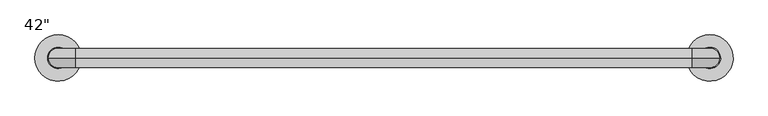
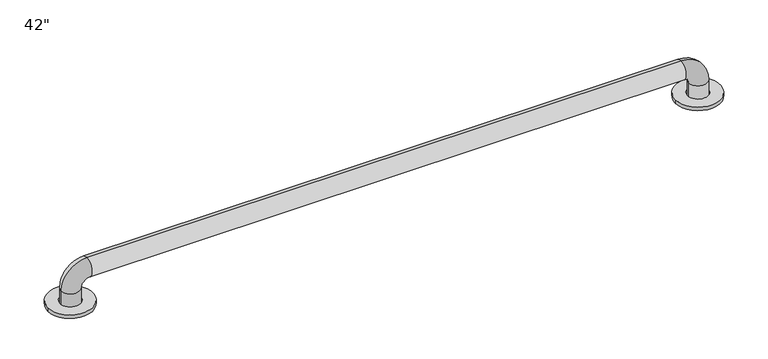
"""IFC4 building model written with IfcOpenShell, lengths in millimetres: proxy geometry."""

import ifcopenshell
import ifcopenshell.guid

model = None  # the IFC model being written
_history = None  # IfcOwnerHistory: only IFC2X3 demands one
_inside = {}  # id of a spatial element -> (the spatial element, [elements in it])
_under = {}  # id of a project, library or spatial element -> (it, [spatial elements below it])
_declared = {}  # id of a project -> (the project, [libraries it declares])
_typed = {}  # id of a type object -> (the type object, [elements of that type])
_made_of = {}  # id of a material, layer set ... -> (it, [elements and type objects made of it])


def new_model(schema):
    """Start an empty IFC model of exactly this schema.

    Asked for "IFC4X3", IfcOpenShell would pick the latest addendum, in which some entities
    have other attributes; the version numbers below select the first issue.
    IFC2X3 requires an IfcOwnerHistory on every rooted entity: one is made here for all.
    """
    global model, _history
    if schema == "IFC4X3":
        model = ifcopenshell.file(schema_version=(4, 3, 0, 0))
    else:
        model = ifcopenshell.file(schema=schema)
    _inside.clear()
    _under.clear()
    _declared.clear()
    _typed.clear()
    _made_of.clear()
    _history = None
    if model.schema == "IFC2X3":
        org = make("IfcOrganization", Name="unknown")
        user = make(
            "IfcPersonAndOrganization",
            ThePerson=make("IfcPerson", FamilyName="unknown"),
            TheOrganization=org,
        )
        app = make(
            "IfcApplication",
            ApplicationDeveloper=org,
            Version="unknown",
            ApplicationFullName="unknown",
            ApplicationIdentifier="unknown",
        )
        _history = make(
            "IfcOwnerHistory",
            OwningUser=user,
            OwningApplication=app,
            ChangeAction="ADDED",
            CreationDate=0,
        )
    return model


def make(cls, **values):
    """One entity of the class cls with the attributes given. An attribute that is None is left unset."""
    return model.create_entity(
        cls, **{name: value for name, value in values.items() if value is not None}
    )


def rooted(cls, **values):
    """An entity with a GlobalId (a new one), such as an element, a storey or a relation."""
    return make(cls, GlobalId=ifcopenshell.guid.new(), OwnerHistory=_history, **values)


def si_unit(unit_type, name, prefix=None):
    """IfcSIUnit, for example si_unit("LENGTHUNIT", "METRE", prefix="MILLI")."""
    return make("IfcSIUnit", UnitType=unit_type, Prefix=prefix, Name=name)


def assignment(units):
    """IfcUnitAssignment: the units of a project."""
    return None if units is None else make("IfcUnitAssignment", Units=units)


def point(xyz):
    """IfcCartesianPoint."""
    return None if xyz is None else make("IfcCartesianPoint", Coordinates=xyz)


def direction(xyz):
    """IfcDirection."""
    return None if xyz is None else make("IfcDirection", DirectionRatios=xyz)


def frame(location, z_axis=None, x_axis=None):
    """IfcAxis2Placement3D, a coordinate frame: its origin and axes. An axis left out is left unset."""
    return make(
        "IfcAxis2Placement3D",
        Location=point(location),
        Axis=direction(z_axis),
        RefDirection=direction(x_axis),
    )


def frame_2d(location, x_axis=None):
    """IfcAxis2Placement2D, a coordinate frame in the plane: its origin and x axis."""
    return make(
        "IfcAxis2Placement2D", Location=point(location), RefDirection=direction(x_axis)
    )


def origin():
    """The frame at (0, 0, 0) with its axes left unset."""
    return frame((0.0, 0.0, 0.0))


def origin_with_axes():
    """The frame at (0, 0, 0) with the z axis (0, 0, 1) and the x axis (1, 0, 0) written out."""
    return frame((0.0, 0.0, 0.0), z_axis=(0.0, 0.0, 1.0), x_axis=(1.0, 0.0, 0.0))


def origin_2d():
    """The frame at (0, 0) in the plane with its x axis left unset."""
    return frame_2d((0.0, 0.0))


def place(relative_to, where):
    """IfcLocalPlacement: puts the frame where relative to a parent placement (None: the world)."""
    return make(
        "IfcLocalPlacement", PlacementRelTo=relative_to, RelativePlacement=where
    )


def context(
    kind, dimensions, precision=None, world=None, true_north=None, identifier=None
):
    """IfcGeometricRepresentationContext, for example the 3D "Model" context."""
    return make(
        "IfcGeometricRepresentationContext",
        ContextIdentifier=identifier,
        ContextType=kind,
        CoordinateSpaceDimension=dimensions,
        Precision=precision,
        WorldCoordinateSystem=world,
        TrueNorth=true_north,
    )


def project(units=None, contexts=None):
    """IfcProject with its units and contexts."""
    return rooted(
        "IfcProject",
        Name="project",
        RepresentationContexts=contexts,
        UnitsInContext=assignment(units),
    )


def spatial(cls, under=None, at=None, **own):
    """A site, building, storey or space (cls), placed at a placement, below another one or the project."""
    s = rooted(cls, ObjectPlacement=at, **own)
    if under is not None:
        _under.setdefault(under.id(), (under, []))[1].append(s)
    return s


def circle_curve(where, radius):
    """IfcCircle in the frame where."""
    return make("IfcCircle", Position=where, Radius=radius)


def ellipse_curve(where, semi_axis1, semi_axis2):
    """IfcEllipse in the frame where."""
    return make(
        "IfcEllipse", Position=where, SemiAxis1=semi_axis1, SemiAxis2=semi_axis2
    )


def trimmed(basis, trim1, trim2, sense, master):
    """IfcTrimmedCurve: the piece of a basis curve between two trims."""
    return make(
        "IfcTrimmedCurve",
        BasisCurve=basis,
        Trim1=trim1,
        Trim2=trim2,
        SenseAgreement=sense,
        MasterRepresentation=master,
    )


def segment(curve, same_sense, transition):
    """IfcCompositeCurveSegment."""
    return make(
        "IfcCompositeCurveSegment",
        Transition=transition,
        SameSense=same_sense,
        ParentCurve=curve,
    )


def composite_curve(segments, self_intersect=None):
    """IfcCompositeCurve: segments joined end to end."""
    return make("IfcCompositeCurve", Segments=segments, SelfIntersect=self_intersect)


def outline(outer, holes=None, kind="AREA"):
    """IfcArbitraryClosedProfileDef: a profile drawn as a closed curve; with holes, ...WithVoids."""
    if holes is None:
        return make("IfcArbitraryClosedProfileDef", ProfileType=kind, OuterCurve=outer)
    return make(
        "IfcArbitraryProfileDefWithVoids",
        ProfileType=kind,
        OuterCurve=outer,
        InnerCurves=holes,
    )


def extrude(swept, where, along, depth):
    """IfcExtrudedAreaSolid: the profile swept, set in the frame where, extruded along a direction by depth."""
    return make(
        "IfcExtrudedAreaSolid",
        SweptArea=swept,
        Position=where,
        ExtrudedDirection=direction(along),
        Depth=depth,
    )


def shape(context_of_items, identifier, shape_type, items):
    """IfcShapeRepresentation: the items that make up one representation, for example the "Body"."""
    return make(
        "IfcShapeRepresentation",
        ContextOfItems=context_of_items,
        RepresentationIdentifier=identifier,
        RepresentationType=shape_type,
        Items=items,
    )


def source(mapping_origin, context_of_items, identifier, shape_type, items):
    """IfcRepresentationMap: a shape defined once, which mapped items show again and again."""
    return make(
        "IfcRepresentationMap",
        MappingOrigin=mapping_origin,
        MappedRepresentation=shape(context_of_items, identifier, shape_type, items),
    )


def transform(
    local_origin,
    x_axis=None,
    y_axis=None,
    z_axis=None,
    scale=None,
    scale2=None,
    scale3=None,
    uniform=True,
):
    """IfcCartesianTransformationOperator3D, or its non-uniform kind. x_axis, y_axis, z_axis: its Axis1, 2, 3."""
    if uniform:
        return make(
            "IfcCartesianTransformationOperator3D",
            Axis1=direction(x_axis),
            Axis2=direction(y_axis),
            LocalOrigin=point(local_origin),
            Scale=scale,
            Axis3=direction(z_axis),
        )
    return make(
        "IfcCartesianTransformationOperator3DnonUniform",
        Axis1=direction(x_axis),
        Axis2=direction(y_axis),
        LocalOrigin=point(local_origin),
        Scale=scale,
        Axis3=direction(z_axis),
        Scale2=scale2,
        Scale3=scale3,
    )


def mapped(mapping_source, mapping_target):
    """IfcMappedItem: shows the shape of a source again, moved by a transform."""
    return make(
        "IfcMappedItem", MappingSource=mapping_source, MappingTarget=mapping_target
    )


def made_of(thing, what):
    """Note that an element or type object is made of a material, layer set ...; save() writes the relation."""
    if what is not None:
        _made_of.setdefault(what.id(), (what, []))[1].append(thing)
    return thing


def element(
    cls,
    number,
    at=None,
    inside=None,
    cuts=None,
    type_object=None,
    material=None,
    context=None,
    identifier="Body",
    shape_type=None,
    held_by="IfcProductDefinitionShape",
    body=None,
    shapes=None,
    **own,
):
    """One element of the class cls, such as IfcWall. Its Tag is "e" and its number.

    at: its placement. inside: the storey or other place that contains it. cuts: it is an
    opening in that element (IfcRelVoidsElement). A single representation is given by context,
    identifier, shape_type and body (its items); several are given by shapes. held_by: the class
    of the entity that holds the representations. save() writes the other relations.
    """
    e = rooted(cls, Tag="e%d" % number, ObjectPlacement=at, **own)
    if body is not None:
        shapes = [shape(context, identifier, shape_type, body)]
    if shapes is not None:
        e.Representation = make(held_by, Representations=shapes)
    if inside is not None:
        _inside.setdefault(inside.id(), (inside, []))[1].append(e)
    if cuts is not None:
        rooted(
            "IfcRelVoidsElement", RelatingBuildingElement=cuts, RelatedOpeningElement=e
        )
    if type_object is not None:
        _typed.setdefault(type_object.id(), (type_object, []))[1].append(e)
    return made_of(e, material)


def aggregate(whole, parts):
    """IfcRelAggregates: a whole, such as a stair, and the parts it consists of."""
    return rooted("IfcRelAggregates", RelatingObject=whole, RelatedObjects=parts)


def save(model, path):
    """Write the relations noted so far, then the file.

    IfcRelAggregates (storeys below a building ...), IfcRelContainedInSpatialStructure (elements
    in a storey), IfcRelDefinesByType, IfcRelAssociatesMaterial and IfcRelDeclares: one each for
    every whole, place, type object, material and project.
    """
    for whole, parts in _under.values():
        aggregate(whole, parts)
    for where, things in _inside.values():
        rooted(
            "IfcRelContainedInSpatialStructure",
            RelatedElements=things,
            RelatingStructure=where,
        )
    for kind, things in _typed.values():
        rooted("IfcRelDefinesByType", RelatedObjects=things, RelatingType=kind)
    for what, things in _made_of.values():
        rooted("IfcRelAssociatesMaterial", RelatedObjects=things, RelatingMaterial=what)
    for by, libraries in _declared.values():
        rooted("IfcRelDeclares", RelatingContext=by, RelatedDefinitions=libraries)
    model.write(path)


def plane_surface(at):
    """IfcPlane: the flat surface through the origin of the frame at, square to its z axis."""
    return make("IfcPlane", Position=at)


def cylinder_surface(at, radius):
    """IfcCylindricalSurface: all points at the distance radius from the z axis of the frame at."""
    return make("IfcCylindricalSurface", Position=at, Radius=radius)


def revolved_surface(curve, axis_point, axis_direction):
    """IfcSurfaceOfRevolution: the curve turned about the line through axis_point along axis_direction."""
    return make(
        "IfcSurfaceOfRevolution",
        SweptCurve=make("IfcArbitraryOpenProfileDef", ProfileType="CURVE", Curve=curve),
        AxisPosition=make("IfcAxis1Placement", Location=point(axis_point), Axis=direction(axis_direction)),
    )


def advanced_brep(points, edges, surfaces, faces):
    """IfcAdvancedBrep: a solid bounded by faces that lie on surfaces and meet in shared edges.

    An edge is (start, end): straight between two places in points (the first is 0);
    or (start, end, curve); or (start, end, curve, False) where it runs against its curve.
    A face is (place in surfaces, loops), or (place, loops, False) where it looks against
    its surface's normal. A loop lists edges by number (the first is 1), with a minus sign
    where the edge is run from its end to its start. The first loop is the outer one.
    """
    corners = [point(p) for p in points]
    vertices = [make("IfcVertexPoint", VertexGeometry=c) for c in corners]
    made = []
    for start, end, *more in edges:
        made.append(
            make(
                "IfcEdgeCurve",
                EdgeStart=vertices[start],
                EdgeEnd=vertices[end],
                EdgeGeometry=more[0] if more else make("IfcPolyline", Points=[corners[start], corners[end]]),
                SameSense=more[1] if len(more) > 1 else True,
            )
        )
    hull = []
    for where, loops, *sense in faces:
        bounds = []
        for j, loop in enumerate(loops):
            ring = [make("IfcOrientedEdge", EdgeElement=made[abs(k) - 1], Orientation=k > 0) for k in loop]
            bounds.append(
                make(
                    "IfcFaceOuterBound" if j == 0 else "IfcFaceBound",
                    Bound=make("IfcEdgeLoop", EdgeList=ring),
                    Orientation=True,
                )
            )
        hull.append(make("IfcAdvancedFace", Bounds=bounds, FaceSurface=surfaces[where], SameSense=sense[0] if sense else True))
    return make("IfcAdvancedBrep", Outer=make("IfcClosedShell", CfsFaces=hull))


def proxy_594e2c3f(model_context):
    return source(origin(), model_context, "Body", "SolidModel", [
        extrude(outline(composite_curve([segment(trimmed(circle_curve(frame_2d((1066.8, 0.0)), 38.1), [point((1028.7, 0.0))], [point((1066.8, 38.1))], False, "CARTESIAN"), True, "CONTINUOUS"), segment(trimmed(circle_curve(frame_2d((1066.8, 0.0)), 38.1), [point((1066.8, 38.1))], [point((1028.7, 0.0))], False, "CARTESIAN"), True, "CONTINUOUS")], self_intersect=False), holes=[composite_curve([segment(trimmed(circle_curve(frame_2d((1066.8, 0.0)), 17.4625), [point((1049.3375, 0.0))], [point((1066.8, 17.4625))], True, "CARTESIAN"), True, "CONTINUOUS"), segment(trimmed(circle_curve(frame_2d((1066.8, 0.0)), 17.4625), [point((1066.8, 17.4625))], [point((1049.3375, 0.0))], True, "CARTESIAN"), True, "CONTINUOUS")], self_intersect=False)]), origin_with_axes(), (0.0, 0.0, 1.0), 6.35),
        extrude(outline(composite_curve([segment(trimmed(circle_curve(origin_2d(), 38.1), [point((-38.1, 0.0))], [point((0.0, 38.1))], False, "CARTESIAN"), True, "CONTINUOUS"), segment(trimmed(circle_curve(origin_2d(), 38.1), [point((0.0, 38.1))], [point((-38.1, 0.0))], False, "CARTESIAN"), True, "CONTINUOUS")], self_intersect=False), holes=[composite_curve([segment(trimmed(circle_curve(origin_2d(), 17.4625), [point((-17.4625, 0.0))], [point((0.0, 17.4625))], True, "CARTESIAN"), True, "CONTINUOUS"), segment(trimmed(circle_curve(origin_2d(), 17.4625), [point((0.0, 17.4625))], [point((-17.4625, 0.0))], True, "CARTESIAN"), True, "CONTINUOUS")], self_intersect=False)]), origin_with_axes(), (0.0, 0.0, 1.0), 6.35),
        advanced_brep(
        [(1082.675, 0.0, 0.0), (1050.925, 0.0, 0.0), (1050.925, 0.0, 28.575), (1082.675, 0.0, 28.575), (1038.225, 0.0, 41.275), (1038.225, 0.0, 73.025), (28.575, 0.0, 41.275), (28.575, 0.0, 73.025), (15.875, 0.0, 28.575), (-15.875, 0.0, 28.575), (-15.875, 0.0, 0.0), (15.875, 0.0, 0.0)],
        [
            (0, 1, circle_curve(frame((1066.8, 0.0, 0.0), z_axis=(0.0, 0.0, -1.0), x_axis=(-1.0, 0.0, 0.0)), 15.875)),
            (1, 0, circle_curve(frame((1066.8, 0.0, 0.0), z_axis=(0.0, 0.0, -1.0), x_axis=(-1.0, 0.0, 0.0)), 15.875)),
            (1, 2),
            (2, 3, circle_curve(frame((1066.8, 0.0, 28.575), z_axis=(0.0, 0.0, -1.0), x_axis=(-1.0, 0.0, 0.0)), 15.875)),
            (3, 0),
            (3, 2, circle_curve(frame((1066.8, 0.0, 28.575), z_axis=(0.0, 0.0, -1.0), x_axis=(-1.0, 0.0, 0.0)), 15.875)),
            (4, 5, circle_curve(frame((1038.225, 0.0, 57.15), z_axis=(1.0, 0.0, 0.0), x_axis=(0.0, 0.0, -1.0)), 15.875)),
            (5, 3, circle_curve(frame((1038.225, 0.0, 28.575), z_axis=(0.0, 1.0, 0.0), x_axis=(1.0, 0.0, 0.0)), 44.45)),
            (2, 4, circle_curve(frame((1038.225, 0.0, 28.575), z_axis=(0.0, -1.0, 0.0), x_axis=(1.0, 0.0, 0.0)), 12.7)),
            (5, 4, circle_curve(frame((1038.225, 0.0, 57.15), z_axis=(1.0, 0.0, 0.0), x_axis=(0.0, 0.0, -1.0)), 15.875)),
            (4, 6),
            (6, 7, circle_curve(frame((28.575, 0.0, 57.15), z_axis=(1.0, 0.0, 0.0), x_axis=(0.0, 0.0, -1.0)), 15.875)),
            (7, 5),
            (7, 6, circle_curve(frame((28.575, 0.0, 57.15), z_axis=(1.0, 0.0, 0.0), x_axis=(0.0, 0.0, -1.0)), 15.875)),
            (8, 9, circle_curve(frame((0.0, 0.0, 28.575), z_axis=(0.0, 0.0, 1.0), x_axis=(1.0, 0.0, 0.0)), 15.875)),
            (9, 7, circle_curve(frame((28.575, 0.0, 28.575), z_axis=(0.0, 1.0, 0.0), x_axis=(0.0, 0.0, 1.0)), 44.45)),
            (6, 8, circle_curve(frame((28.575, 0.0, 28.575), z_axis=(0.0, -1.0, 0.0), x_axis=(0.0, 0.0, 1.0)), 12.7)),
            (9, 8, circle_curve(frame((0.0, 0.0, 28.575), z_axis=(0.0, 0.0, 1.0), x_axis=(1.0, 0.0, 0.0)), 15.875)),
            (10, 11, circle_curve(frame((0.0, 0.0, 0.0), z_axis=(0.0, 0.0, -1.0), x_axis=(1.0, 0.0, 0.0)), 15.875)),
            (11, 10, circle_curve(frame((0.0, 0.0, 0.0), z_axis=(0.0, 0.0, -1.0), x_axis=(1.0, 0.0, 0.0)), 15.875)),
            (8, 11),
            (10, 9),
        ],
        [
            plane_surface(frame((1066.8, 0.0, 0.0), z_axis=(0.0, 0.0, -1.0), x_axis=(0.0, 1.0, 0.0))),
            cylinder_surface(frame((1066.8, 0.0, 0.0), z_axis=(0.0, 0.0, -1.0), x_axis=(-1.0, 0.0, 0.0)), 15.875),
            revolved_surface(trimmed(ellipse_curve(frame((1066.8, 0.0, 28.575), z_axis=(0.0, 0.0, 1.0), x_axis=(-1.0, 0.0, 0.0)), 15.875, 15.875), [point((1082.675, 0.0, 28.575))], [point((1050.925, 0.0, 28.575))], True, "CARTESIAN"), (1038.225, 0.0, 28.575), (0.0, 1.0, 0.0)),
            revolved_surface(trimmed(ellipse_curve(frame((1066.8, 0.0, 28.575), z_axis=(0.0, 0.0, 1.0), x_axis=(-1.0, 0.0, 0.0)), 15.875, 15.875), [point((1050.925, 0.0, 28.575))], [point((1082.675, 0.0, 28.575))], True, "CARTESIAN"), (1038.225, 0.0, 28.575), (0.0, 1.0, 0.0)),
            cylinder_surface(frame((1038.225, 0.0, 57.15), z_axis=(1.0, 0.0, 0.0), x_axis=(0.0, 0.0, -1.0)), 15.875),
            revolved_surface(trimmed(ellipse_curve(frame((28.575, 0.0, 57.15), z_axis=(-1.0, 0.0, 0.0), x_axis=(0.0, 0.0, -1.0)), 15.875, 15.875), [point((28.575, 0.0, 73.025))], [point((28.575, 0.0, 41.275))], True, "CARTESIAN"), (28.575, 0.0, 28.575), (0.0, 1.0, 0.0)),
            revolved_surface(trimmed(ellipse_curve(frame((28.575, 0.0, 57.15), z_axis=(-1.0, 0.0, 0.0), x_axis=(0.0, 0.0, -1.0)), 15.875, 15.875), [point((28.575, 0.0, 41.275))], [point((28.575, 0.0, 73.025))], True, "CARTESIAN"), (28.575, 0.0, 28.575), (0.0, 1.0, 0.0)),
            plane_surface(frame((0.0, 0.0, 0.0), z_axis=(0.0, 0.0, -1.0), x_axis=(0.0, 1.0, 0.0))),
            cylinder_surface(frame((0.0, 0.0, 28.575), z_axis=(0.0, 0.0, 1.0), x_axis=(1.0, 0.0, 0.0)), 15.875),
        ],
        [
            (0, [[1, 2]]),
            (1, [[3, 4, 5, -2]]),
            (1, [[-5, 6, -3, -1]]),
            (2, [[7, 8, -4, 9]]),
            (3, [[10, -9, -6, -8]]),
            (4, [[11, 12, 13, -7]]),
            (4, [[-13, 14, -11, -10]]),
            (5, [[15, 16, -12, 17]]),
            (6, [[18, -17, -14, -16]]),
            (7, [[19, 20]]),
            (8, [[21, -19, 22, -15]]),
            (8, [[-22, -20, -21, -18]]),
        ],
    ),
    ])


if __name__ == "__main__":
    model = new_model("IFC4")
    model_context = context("Model", 3, world=origin())
    ifc_project = project(units=[si_unit("LENGTHUNIT", "METRE", prefix="MILLI")], contexts=[model_context])
    site = spatial("IfcSite", under=ifc_project)
    building = spatial("IfcBuilding", under=site)
    placement = place(None, origin())
    proxy_shape = proxy_594e2c3f(model_context)
    element("IfcBuildingElementProxy", 1, Name="Seqm-Grab Bar : 42\"", ObjectType="Seqm-Grab Bar : 42\"", at=placement, inside=building, context=model_context, shape_type="MappedRepresentation", body=[
        mapped(proxy_shape, transform((0.0, 0.0, 0.0), x_axis=(1.0, 0.0, 0.0), y_axis=(0.0, 1.0, 0.0), z_axis=(0.0, 0.0, 1.0))),
    ])
    save(model, "model.ifc")

# Revit data of these elements
# Type "Seqm-Grab Bar : 42\""
#   Spec Number = "10 28 00"
#   Spec Description = "42\" GRAB BAR"
#   Length = 3' - 6"
#   Default Elevation = 4' - 0"
#   Grab Bar Material = GRAB BARS - AT ADA RESTROOMS ONLY
# Element 1 (IfcBuildingElementProxy, "Seqm-Grab Bar : 42\"")
#   Materials on its faces: "GRAB BARS - AT ADA RESTROOMS ONLY"
# Materials
#   "GRAB BARS - AT ADA RESTROOMS ONLY": class "Generic", colour RGB 120 120 120, transparency 0, Cost = 0
